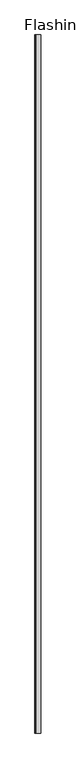
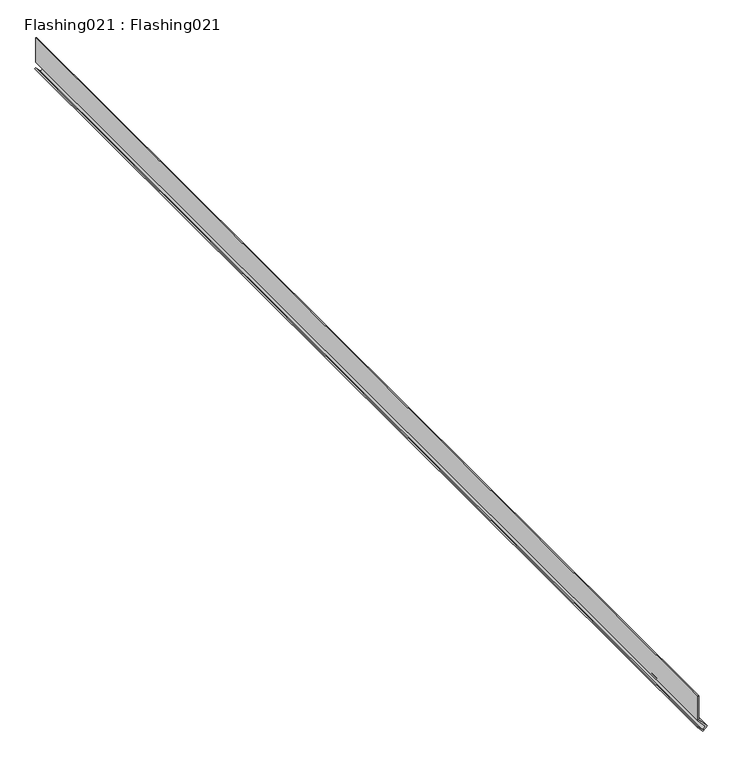
"""IFC4 building model written with IfcOpenShell, lengths in millimetres: proxy geometry, Flashing021 : Flashing021."""

from ifc_helpers import new_model, si_unit, frame, origin, place, context, project, spatial, polyline, outline, extrude, source, transform, mapped, element, save


def flashing021_flashing021_f64f48d8(model_context):
    return source(origin(), model_context, "Body", "SweptSolid", [
        extrude(outline(polyline([(43008.8710938, 16651.7480469), (42993.6445313, 16665.2148438), (42989.0546875, 16660.4316406), (42998.2304688, 16652.1347656), (42996.8890886, 16650.6512902), (42986.1852076, 16660.3298953), (42993.5310498, 16667.9852007), (43009.6286352, 16653.7480469), (43053.53125, 16653.7480469), (43053.53125, 16651.7480469), (43008.8710938, 16651.7480469)])), frame((0.0, 7982.1435673, 0.0), z_axis=(0.0, 1.0, 0.0), x_axis=(0.0, 0.0, 1.0)), (0.0, 0.0, 1.0), 2000.0),
    ])


if __name__ == "__main__":
    model = new_model("IFC4")
    model_context = context("Model", 3, world=origin())
    ifc_project = project(units=[si_unit("LENGTHUNIT", "METRE", prefix="MILLI")], contexts=[model_context])
    site = spatial("IfcSite", under=ifc_project)
    building = spatial("IfcBuilding", under=site)
    placement = place(None, origin())
    flashing021_flashing021_shape = flashing021_flashing021_f64f48d8(model_context)
    element("IfcBuildingElementProxy", 1, Name="Flashing021 : Flashing021", ObjectType="Flashing021 : Flashing021", at=placement, inside=building, context=model_context, shape_type="MappedRepresentation", body=[
        mapped(flashing021_flashing021_shape, transform((0.0, 0.0, 0.0), x_axis=(1.0, 0.0, 0.0), y_axis=(0.0, 1.0, 0.0), z_axis=(0.0, 0.0, 1.0))),
    ])
    save(model, "model.ifc")

# Revit data of these elements
# Type "Flashing021 : Flashing021"
#   NameOverride = "Flashing021"
# Element 1 (IfcBuildingElementProxy, "Flashing021 : Flashing021")
#   Materials on its faces: "16GA. COPPER BRAKE METAL FLASHING"
# Materials
#   "16GA. COPPER BRAKE METAL FLASHING": class "Unassigned", colour RGB 128 128 128, transparency 0, Cost = 0
